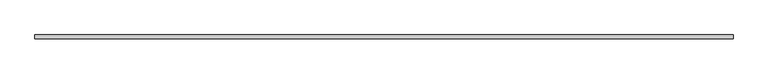
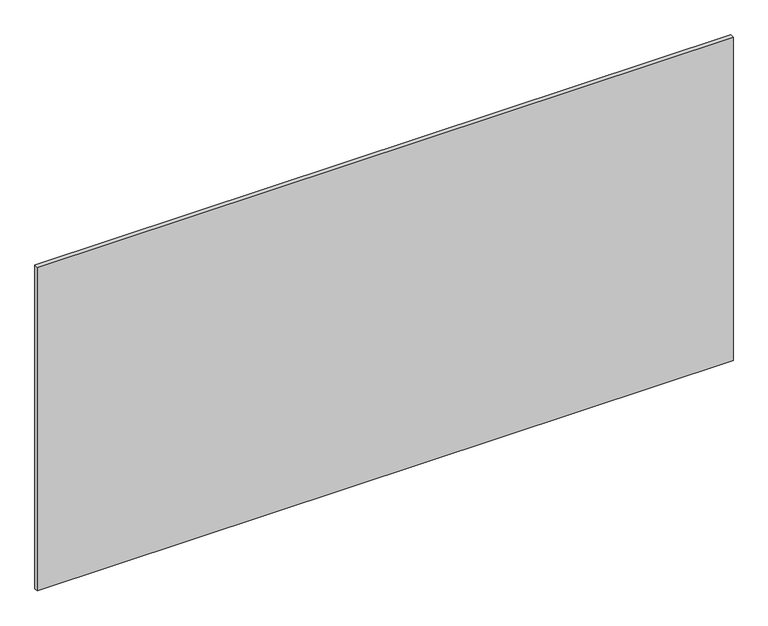
"""IFC4 building model written with IfcOpenShell, lengths in millimetres: railing geometry, ML_Painéis2 : ML_Painéis."""

from ifc_helpers import new_model, si_unit, frame, origin, place, context, project, spatial, polyline, outline, extrude, source, transform, mapped, element, save


def railing_17c90805(model_context):
    return source(origin(), model_context, "Body", "SweptSolid", [
        extrude(outline(polyline([(-4674.5702584, 2133.3602771), (-4674.5702584, 2121.3602771), (-6910.5702584, 2121.3602771), (-6910.5702584, 2133.3602771), (-4674.5702584, 2133.3602771)])), frame((0.0, 0.0, 4122.0679199), z_axis=(0.0, 0.0, 1.0), x_axis=(1.0, 0.0, 0.0)), (0.0, 0.0, 1.0), 1100.0),
    ])


if __name__ == "__main__":
    model = new_model("IFC4")
    model_context = context("Model", 3, world=origin())
    ifc_project = project(units=[si_unit("LENGTHUNIT", "METRE", prefix="MILLI")], contexts=[model_context])
    site = spatial("IfcSite", under=ifc_project)
    building = spatial("IfcBuilding", under=site)
    placement = place(None, origin())
    railing_shape = railing_17c90805(model_context)
    element("IfcRailing", 1, ObjectType="ML_Painéis2 : ML_Painéis", at=placement, inside=building, context=model_context, shape_type="MappedRepresentation", body=[
        mapped(railing_shape, transform((0.0, 0.0, 0.0), x_axis=(1.0, 0.0, 0.0), y_axis=(0.0, 1.0, 0.0), z_axis=(0.0, 0.0, 1.0))),
    ])
    save(model, "model.ifc")

# Revit data of these elements
# Type "ML_Painéis2 : ML_Painéis"
#   ME_Área [instance default] = 2.4596 m²
#   ME_Espessura [instance default] = 0.012 m
#   ME_Dist Painéis [instance default] = 0.002 m
#   ME_Compr Painéis [instance default] = 2.236 m
#   ME_Compr [instance default] = 2.24 m
#   ME_Altura [instance default] = 1.10 m
#   ME_Quant Painéis [instance default] = 3
#   ME_Painel Único [instance default] = yes
#   ME_Paineis Vários [instance default] = no
#   ME_Material Tipo Vidro [instance default] = .VIDRO GENÉRICO
# Element 1 (IfcRailing, "ML_Painéis2 : ML_Painéis")
#   Materials on its faces: ".VIDRO GENÉRICO"
# Materials
#   ".VIDRO GENÉRICO": class ".CC_VIDRO", colour RGB 0 128 192, transparency 0.9, Description = "Vidro comum", Cost = 0
